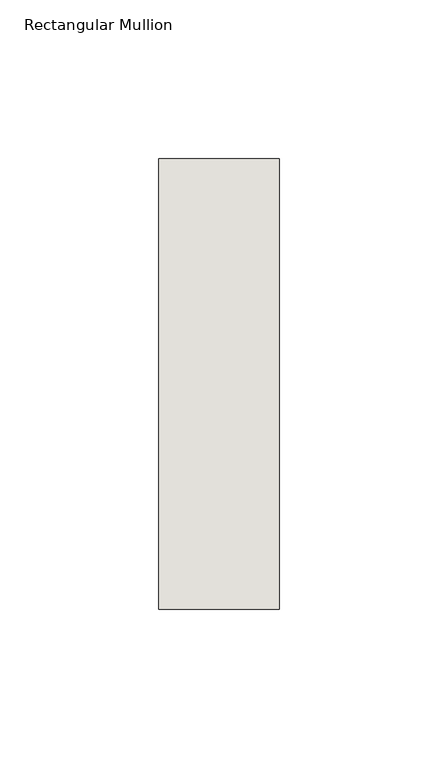
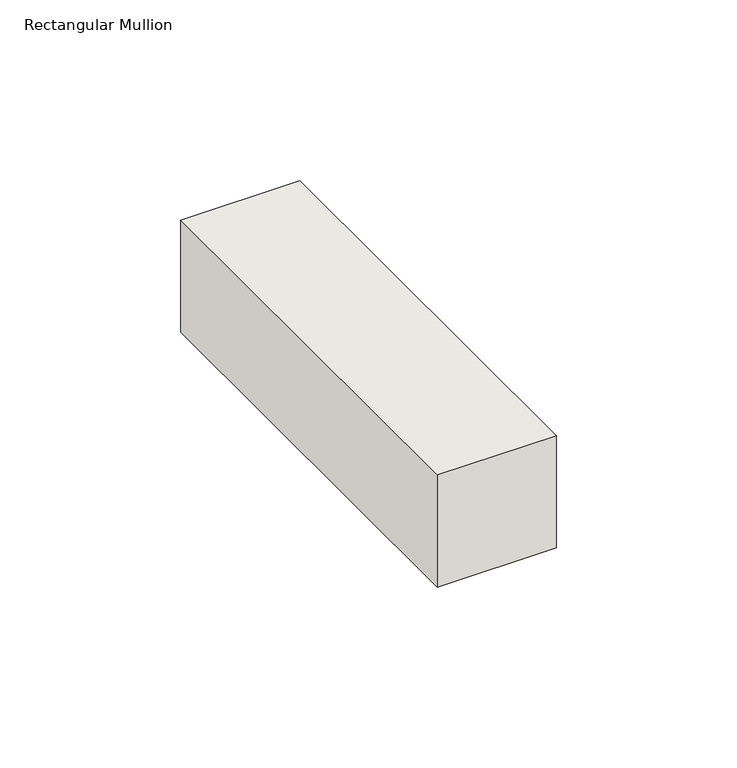
"""IFC4 building model written with IfcOpenShell, lengths in millimetres: wall geometry, Rectangular Mullion : NLRS_21_CWM_hsb-regel 38x142_gen_rsf."""

from ifc_helpers import new_model, si_unit, frame, origin, place, context, project, spatial, polyline, outline, extrude, source, transform, mapped, element, save


def rectangular_mullion_c09c4bb1(model_context):
    return source(origin(), model_context, "Body", "SweptSolid", [
        extrude(outline(polyline([(19.0, -71.0), (-19.0, -71.0), (-19.0, 71.0), (19.0, 71.0), (19.0, -71.0)])), frame((0.0, 0.0, -38.0), z_axis=(0.0, 0.0, 1.0), x_axis=(1.0, 0.0, 0.0)), (0.0, 0.0, 1.0), 38.0),
    ])


if __name__ == "__main__":
    model = new_model("IFC4")
    model_context = context("Model", 3, world=origin())
    ifc_project = project(units=[si_unit("LENGTHUNIT", "METRE", prefix="MILLI")], contexts=[model_context])
    site = spatial("IfcSite", under=ifc_project)
    building = spatial("IfcBuilding", under=site)
    placement = place(None, origin())
    rectangular_mullion_shape = rectangular_mullion_c09c4bb1(model_context)
    element("IfcWall", 1, ObjectType="Rectangular Mullion : NLRS_21_CWM_hsb-regel 38x142_gen_rsf", at=placement, inside=building, context=model_context, shape_type="MappedRepresentation", body=[
        mapped(rectangular_mullion_shape, transform((0.0, 0.0, 0.0), x_axis=(1.0, 0.0, 0.0), y_axis=(0.0, 1.0, 0.0), z_axis=(0.0, 0.0, 1.0))),
    ])
    save(model, "model.ifc")

# Revit data of these elements
# Type "Rectangular Mullion : NLRS_21_CWM_hsb-regel 38x142_gen_rsf"
#   Type IfcGUID = "07M7mRoiH1CR8m_RSKIwpF"
#   Assembly Code = "21.10"
#   IfcExportAs = "IfcWall"
#   built-in parameter 1007322 = 0.465879 (stored number, unit not read)
#   built-in parameter 1007321 = 0.062336 (stored number, unit not read)
#   built-in parameter 1007320 = 0.062336 (stored number, unit not read)
# Element 1 (IfcWall, "Rectangular Mullion : NLRS_21_CWM_hsb-regel 38x142_gen_rsf")
#   Materials on its faces: "NLRS_i2_hout naaldhout vuren_gen_rsf"
# Materials
#   "NLRS_i2_hout naaldhout vuren_gen_rsf": class "I - Hout", colour RGB 234 199 147, transparency 0, Keynote = "i2", Manufacturer = "Revit Standards Foundation", URL = "www.revitstandards.org", Description = "hout vuren", Cost = 0
